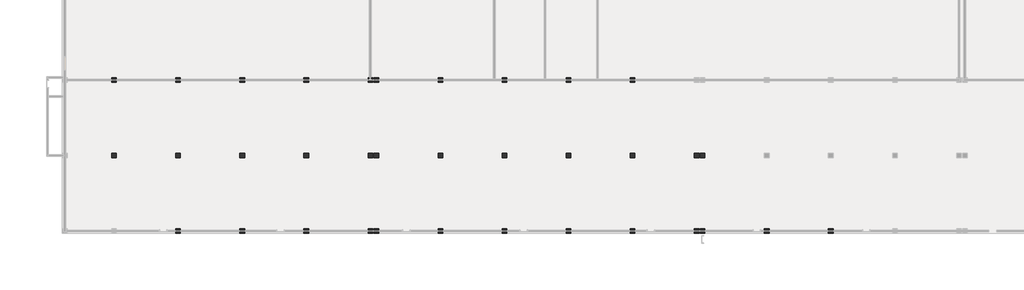
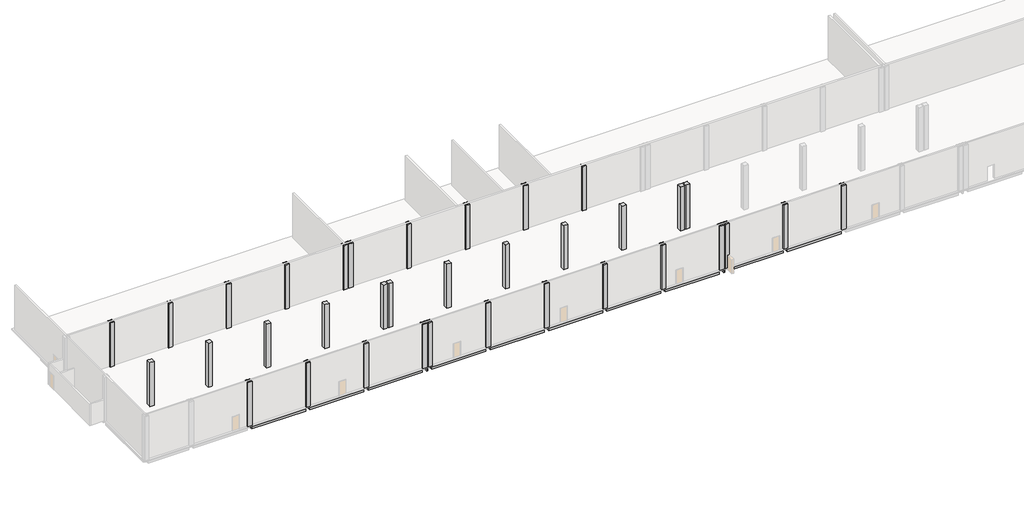
# One storey, part 2 of 4: 35 columns, 12 beams.
"""IFC4 building model written with IfcOpenShell, lengths in millimetres."""

import ifcopenshell
import ifcopenshell.guid

model = None  # the IFC model being written
_history = None  # IfcOwnerHistory: only IFC2X3 demands one
_inside = {}  # id of a spatial element -> (the spatial element, [elements in it])
_under = {}  # id of a project, library or spatial element -> (it, [spatial elements below it])
_declared = {}  # id of a project -> (the project, [libraries it declares])
_typed = {}  # id of a type object -> (the type object, [elements of that type])
_made_of = {}  # id of a material, layer set ... -> (it, [elements and type objects made of it])


def new_model(schema):
    """Start an empty IFC model of exactly this schema.

    Asked for "IFC4X3", IfcOpenShell would pick the latest addendum, in which some entities
    have other attributes; the version numbers below select the first issue.
    IFC2X3 requires an IfcOwnerHistory on every rooted entity: one is made here for all.
    """
    global model, _history
    if schema == "IFC4X3":
        model = ifcopenshell.file(schema_version=(4, 3, 0, 0))
    else:
        model = ifcopenshell.file(schema=schema)
    _inside.clear()
    _under.clear()
    _declared.clear()
    _typed.clear()
    _made_of.clear()
    _history = None
    if model.schema == "IFC2X3":
        org = make("IfcOrganization", Name="unknown")
        user = make(
            "IfcPersonAndOrganization",
            ThePerson=make("IfcPerson", FamilyName="unknown"),
            TheOrganization=org,
        )
        app = make(
            "IfcApplication",
            ApplicationDeveloper=org,
            Version="unknown",
            ApplicationFullName="unknown",
            ApplicationIdentifier="unknown",
        )
        _history = make(
            "IfcOwnerHistory",
            OwningUser=user,
            OwningApplication=app,
            ChangeAction="ADDED",
            CreationDate=0,
        )
    return model


def make(cls, **values):
    """One entity of the class cls with the attributes given. An attribute that is None is left unset."""
    return model.create_entity(
        cls, **{name: value for name, value in values.items() if value is not None}
    )


def rooted(cls, **values):
    """An entity with a GlobalId (a new one), such as an element, a storey or a relation."""
    return make(cls, GlobalId=ifcopenshell.guid.new(), OwnerHistory=_history, **values)


def si_unit(unit_type, name, prefix=None):
    """IfcSIUnit, for example si_unit("LENGTHUNIT", "METRE", prefix="MILLI")."""
    return make("IfcSIUnit", UnitType=unit_type, Prefix=prefix, Name=name)


def assignment(units):
    """IfcUnitAssignment: the units of a project."""
    return None if units is None else make("IfcUnitAssignment", Units=units)


def point(xyz):
    """IfcCartesianPoint."""
    return None if xyz is None else make("IfcCartesianPoint", Coordinates=xyz)


def direction(xyz):
    """IfcDirection."""
    return None if xyz is None else make("IfcDirection", DirectionRatios=xyz)


def frame(location, z_axis=None, x_axis=None):
    """IfcAxis2Placement3D, a coordinate frame: its origin and axes. An axis left out is left unset."""
    return make(
        "IfcAxis2Placement3D",
        Location=point(location),
        Axis=direction(z_axis),
        RefDirection=direction(x_axis),
    )


def origin():
    """The frame at (0, 0, 0) with its axes left unset."""
    return frame((0.0, 0.0, 0.0))


def place(relative_to, where):
    """IfcLocalPlacement: puts the frame where relative to a parent placement (None: the world)."""
    return make(
        "IfcLocalPlacement", PlacementRelTo=relative_to, RelativePlacement=where
    )


def context(
    kind, dimensions, precision=None, world=None, true_north=None, identifier=None
):
    """IfcGeometricRepresentationContext, for example the 3D "Model" context."""
    return make(
        "IfcGeometricRepresentationContext",
        ContextIdentifier=identifier,
        ContextType=kind,
        CoordinateSpaceDimension=dimensions,
        Precision=precision,
        WorldCoordinateSystem=world,
        TrueNorth=true_north,
    )


def project(units=None, contexts=None):
    """IfcProject with its units and contexts."""
    return rooted(
        "IfcProject",
        Name="project",
        RepresentationContexts=contexts,
        UnitsInContext=assignment(units),
    )


def spatial(cls, under=None, at=None, **own):
    """A site, building, storey or space (cls), placed at a placement, below another one or the project."""
    s = rooted(cls, ObjectPlacement=at, **own)
    if under is not None:
        _under.setdefault(under.id(), (under, []))[1].append(s)
    return s


def polyline(points):
    """IfcPolyline through the points."""
    return make("IfcPolyline", Points=[point(p) for p in points])


def outline(outer, holes=None, kind="AREA"):
    """IfcArbitraryClosedProfileDef: a profile drawn as a closed curve; with holes, ...WithVoids."""
    if holes is None:
        return make("IfcArbitraryClosedProfileDef", ProfileType=kind, OuterCurve=outer)
    return make(
        "IfcArbitraryProfileDefWithVoids",
        ProfileType=kind,
        OuterCurve=outer,
        InnerCurves=holes,
    )


def extrude(swept, where, along, depth):
    """IfcExtrudedAreaSolid: the profile swept, set in the frame where, extruded along a direction by depth."""
    return make(
        "IfcExtrudedAreaSolid",
        SweptArea=swept,
        Position=where,
        ExtrudedDirection=direction(along),
        Depth=depth,
    )


def faces_of(points, faces, orient=None, outer=None):
    """IfcFace entities. A face is a list of loops; a loop is a list of indices into points, from 0.

    orient and outer hold one flag for each loop. By default every Orientation is true, the
    first loop of a face is its IfcFaceOuterBound and the others are IfcFaceBound.
    """
    made = []
    for i, loops in enumerate(faces):
        bounds = []
        for j, loop in enumerate(loops):
            is_outer = j == 0 if outer is None else outer[i][j]
            bounds.append(
                make(
                    "IfcFaceOuterBound" if is_outer else "IfcFaceBound",
                    Bound=make("IfcPolyLoop", Polygon=[points[k] for k in loop]),
                    Orientation=True if orient is None else orient[i][j],
                )
            )
        made.append(make("IfcFace", Bounds=bounds))
    return made


def faceted_brep(points, faces, orient=None, outer=None, voids=None):
    """IfcFacetedBrep: a solid bounded by flat faces; with voids (closed shells), ...WithVoids."""
    shared = [point(p) for p in points]
    hull = make("IfcClosedShell", CfsFaces=faces_of(shared, faces, orient, outer))
    if voids is None:
        return make("IfcFacetedBrep", Outer=hull)
    return make(
        "IfcFacetedBrepWithVoids",
        Outer=hull,
        Voids=[
            make(cls, CfsFaces=faces_of(shared, fs, o, b)) for cls, fs, o, b in voids
        ],
    )


def shape(context_of_items, identifier, shape_type, items):
    """IfcShapeRepresentation: the items that make up one representation, for example the "Body"."""
    return make(
        "IfcShapeRepresentation",
        ContextOfItems=context_of_items,
        RepresentationIdentifier=identifier,
        RepresentationType=shape_type,
        Items=items,
    )


def made_of(thing, what):
    """Note that an element or type object is made of a material, layer set ...; save() writes the relation."""
    if what is not None:
        _made_of.setdefault(what.id(), (what, []))[1].append(thing)
    return thing


def element(
    cls,
    number,
    at=None,
    inside=None,
    cuts=None,
    type_object=None,
    material=None,
    context=None,
    identifier="Body",
    shape_type=None,
    held_by="IfcProductDefinitionShape",
    body=None,
    shapes=None,
    **own,
):
    """One element of the class cls, such as IfcWall. Its Tag is "e" and its number.

    at: its placement. inside: the storey or other place that contains it. cuts: it is an
    opening in that element (IfcRelVoidsElement). A single representation is given by context,
    identifier, shape_type and body (its items); several are given by shapes. held_by: the class
    of the entity that holds the representations. save() writes the other relations.
    """
    e = rooted(cls, Tag="e%d" % number, ObjectPlacement=at, **own)
    if body is not None:
        shapes = [shape(context, identifier, shape_type, body)]
    if shapes is not None:
        e.Representation = make(held_by, Representations=shapes)
    if inside is not None:
        _inside.setdefault(inside.id(), (inside, []))[1].append(e)
    if cuts is not None:
        rooted(
            "IfcRelVoidsElement", RelatingBuildingElement=cuts, RelatedOpeningElement=e
        )
    if type_object is not None:
        _typed.setdefault(type_object.id(), (type_object, []))[1].append(e)
    return made_of(e, material)


def aggregate(whole, parts):
    """IfcRelAggregates: a whole, such as a stair, and the parts it consists of."""
    return rooted("IfcRelAggregates", RelatingObject=whole, RelatedObjects=parts)


def save(model, path):
    """Write the relations noted so far, then the file.

    IfcRelAggregates (storeys below a building ...), IfcRelContainedInSpatialStructure (elements
    in a storey), IfcRelDefinesByType, IfcRelAssociatesMaterial and IfcRelDeclares: one each for
    every whole, place, type object, material and project.
    """
    for whole, parts in _under.values():
        aggregate(whole, parts)
    for where, things in _inside.values():
        rooted(
            "IfcRelContainedInSpatialStructure",
            RelatedElements=things,
            RelatingStructure=where,
        )
    for kind, things in _typed.values():
        rooted("IfcRelDefinesByType", RelatedObjects=things, RelatingType=kind)
    for what, things in _made_of.values():
        rooted("IfcRelAssociatesMaterial", RelatedObjects=things, RelatingMaterial=what)
    for by, libraries in _declared.values():
        rooted("IfcRelDeclares", RelatingContext=by, RelatedDefinitions=libraries)
    model.write(path)


model = new_model("IFC4")

# Units and contexts
model_context = context("Model", 3, world=origin())
ifc_project = project(units=[si_unit("LENGTHUNIT", "METRE", prefix="MILLI")], contexts=[model_context])

# Site, building, storey
site = spatial("IfcSite", under=ifc_project)
building = spatial("IfcBuilding", under=site)
storey = spatial("IfcBuildingStorey", under=building, Name="01_T.O.F", Elevation=299.9618634)

# Beams
placement = place(None, origin())
element("IfcBeam", 1, ObjectType="RC Beam_Rectangular : H_SB_AR_S16_TG_B400xH600", at=placement, inside=storey, context=model_context, shape_type="SweptSolid", body=[
    extrude(outline(polyline([(10430.0, -25475.4791411), (10430.0, -25125.4791411), (18030.0, -25125.4791411), (18030.0, -25475.4791411), (10430.0, -25475.4791411)])), frame((0.0, 0.0, -300.0381366), z_axis=(0.0, 0.0, 1.0), x_axis=(1.0, 0.0, 0.0)), (0.0, 0.0, 1.0), 450.0),
])
element("IfcBeam", 2, ObjectType="RC Beam_Rectangular : H_SB_AR_S16_TG_B400xH600", at=placement, inside=storey, context=model_context, shape_type="SweptSolid", body=[
    extrude(outline(polyline([(18630.0, -25475.4791411), (18630.0, -25125.4791411), (26230.0, -25125.4791411), (26230.0, -25475.4791411), (18630.0, -25475.4791411)])), frame((0.0, 0.0, -300.0381366), z_axis=(0.0, 0.0, 1.0), x_axis=(1.0, 0.0, 0.0)), (0.0, 0.0, 1.0), 450.0),
])
element("IfcBeam", 3, ObjectType="RC Beam_Rectangular : H_SB_AR_S16_TG_B400xH600", at=placement, inside=storey, context=model_context, shape_type="SweptSolid", body=[
    extrude(outline(polyline([(26830.0, -25475.4791411), (26830.0, -25125.4791411), (34430.0, -25125.4791411), (34430.0, -25475.4791411), (26830.0, -25475.4791411)])), frame((0.0, 0.0, -300.0381366), z_axis=(0.0, 0.0, 1.0), x_axis=(1.0, 0.0, 0.0)), (0.0, 0.0, 1.0), 450.0),
])
element("IfcBeam", 4, ObjectType="RC Beam_Rectangular : H_SB_AR_S16_TG_B400xH600", at=placement, inside=storey, context=model_context, shape_type="SweptSolid", body=[
    extrude(outline(polyline([(35030.0, -25475.4791411), (35030.0, -25125.4791411), (35180.0, -25125.4791411), (35180.0, -25475.4791411), (35030.0, -25475.4791411)])), frame((0.0, 0.0, -300.0381366), z_axis=(0.0, 0.0, 1.0), x_axis=(1.0, 0.0, 0.0)), (0.0, 0.0, 1.0), 450.0),
])
element("IfcBeam", 5, ObjectType="RC Beam_Rectangular : H_SB_AR_S16_TG_B400xH600", at=placement, inside=storey, context=model_context, shape_type="SweptSolid", body=[
    extrude(outline(polyline([(35780.0, -25475.4791411), (35780.0, -25125.4791411), (43380.0, -25125.4791411), (43380.0, -25475.4791411), (35780.0, -25475.4791411)])), frame((0.0, 0.0, -300.0381366), z_axis=(0.0, 0.0, 1.0), x_axis=(1.0, 0.0, 0.0)), (0.0, 0.0, 1.0), 450.0),
])
element("IfcBeam", 6, ObjectType="RC Beam_Rectangular : H_SB_AR_S16_TG_B400xH600", at=placement, inside=storey, context=model_context, shape_type="SweptSolid", body=[
    extrude(outline(polyline([(43980.0, -25475.4791411), (43980.0, -25125.4791411), (51580.0, -25125.4791411), (51580.0, -25475.4791411), (43980.0, -25475.4791411)])), frame((0.0, 0.0, -300.0381366), z_axis=(0.0, 0.0, 1.0), x_axis=(1.0, 0.0, 0.0)), (0.0, 0.0, 1.0), 450.0),
])
element("IfcBeam", 7, ObjectType="RC Beam_Rectangular : H_SB_AR_S16_TG_B400xH600", at=placement, inside=storey, context=model_context, shape_type="SweptSolid", body=[
    extrude(outline(polyline([(52180.0, -25475.4791411), (52180.0, -25125.4791411), (59780.0, -25125.4791411), (59780.0, -25475.4791411), (52180.0, -25475.4791411)])), frame((0.0, 0.0, -300.0381366), z_axis=(0.0, 0.0, 1.0), x_axis=(1.0, 0.0, 0.0)), (0.0, 0.0, 1.0), 450.0),
])
element("IfcBeam", 8, ObjectType="RC Beam_Rectangular : H_SB_AR_S16_TG_B400xH600", at=placement, inside=storey, context=model_context, shape_type="SweptSolid", body=[
    extrude(outline(polyline([(60380.0, -25475.4791411), (60380.0, -25125.4791411), (67980.0, -25125.4791411), (67980.0, -25475.4791411), (60380.0, -25475.4791411)])), frame((0.0, 0.0, -300.0381366), z_axis=(0.0, 0.0, 1.0), x_axis=(1.0, 0.0, 0.0)), (0.0, 0.0, 1.0), 450.0),
])
element("IfcBeam", 9, ObjectType="RC Beam_Rectangular : H_SB_AR_S16_TG_B400xH600", at=placement, inside=storey, context=model_context, shape_type="SweptSolid", body=[
    extrude(outline(polyline([(68580.0, -25475.4791411), (68580.0, -25125.4791411), (76180.0, -25125.4791411), (76180.0, -25475.4791411), (68580.0, -25475.4791411)])), frame((0.0, 0.0, -300.0381366), z_axis=(0.0, 0.0, 1.0), x_axis=(1.0, 0.0, 0.0)), (0.0, 0.0, 1.0), 450.0),
])
element("IfcBeam", 10, ObjectType="RC Beam_Rectangular : H_SB_AR_S16_TG_B400xH600", at=placement, inside=storey, context=model_context, shape_type="SweptSolid", body=[
    extrude(outline(polyline([(76780.0, -25475.4791411), (76780.0, -25125.4791411), (76930.0, -25125.4791411), (76930.0, -25475.4791411), (76780.0, -25475.4791411)])), frame((0.0, 0.0, -300.0381366), z_axis=(0.0, 0.0, 1.0), x_axis=(1.0, 0.0, 0.0)), (0.0, 0.0, 1.0), 450.0),
])
element("IfcBeam", 11, ObjectType="RC Beam_Rectangular : H_SB_AR_S16_TG_B400xH600", at=placement, inside=storey, context=model_context, shape_type="SweptSolid", body=[
    extrude(outline(polyline([(77530.0, -25475.4791411), (77530.0, -25125.4791411), (85130.0, -25125.4791411), (85130.0, -25475.4791411), (77530.0, -25475.4791411)])), frame((0.0, 0.0, -300.0381366), z_axis=(0.0, 0.0, 1.0), x_axis=(1.0, 0.0, 0.0)), (0.0, 0.0, 1.0), 450.0),
])
element("IfcBeam", 12, ObjectType="RC Beam_Rectangular : H_SB_AR_S16_TG_B400xH600", at=placement, inside=storey, context=model_context, shape_type="SweptSolid", body=[
    extrude(outline(polyline([(85730.0, -25475.4791411), (85730.0, -25125.4791411), (93330.0, -25125.4791411), (93330.0, -25475.4791411), (85730.0, -25475.4791411)])), frame((0.0, 0.0, -300.0381366), z_axis=(0.0, 0.0, 1.0), x_axis=(1.0, 0.0, 0.0)), (0.0, 0.0, 1.0), 450.0),
])

# Columns
element("IfcColumn", 13, ObjectType="RC_Column_Rectangular : H_SC_AR_S15_W600xL600", at=placement, inside=storey, context=model_context, shape_type="Brep", body=[
    faceted_brep([(2230.0, -5700.4791411, 299.9618634), (2230.0, -6300.4791411, 299.9618634), (1630.0, -6300.4791411, 299.9618634), (1630.0, -5700.4791411, 299.9618634), (2230.0, -5700.4791411, 6848.9618634), (2230.0, -5850.4791411, 6848.9618634), (2230.0, -6150.4791411, 6848.9618634), (2230.0, -6300.4791411, 6848.9618634), (2080.0, -6300.4791411, 6848.9618634), (1780.0, -6300.4791411, 6848.9618634), (1630.0, -6300.4791411, 6848.9618634), (1630.0, -6150.4791411, 6848.9618634), (1630.0, -5850.4791411, 6848.9618634), (1630.0, -5700.4791411, 6848.9618634), (1780.0, -5700.4791411, 6848.9618634), (2080.0, -5700.4791411, 6848.9618634)], [[[0, 1, 2, 3]], [[1, 0, 4, 5, 6, 7]], [[2, 1, 7, 8, 9, 10]], [[3, 2, 10, 11, 12, 13]], [[0, 3, 13, 14, 15, 4]], [[7, 6, 5, 4, 15, 14, 13, 12, 11, 10, 9, 8]]]),
])
element("IfcColumn", 14, ObjectType="RC_Column_Rectangular : H_SC_AR_S15_W600xL600", at=placement, inside=storey, context=model_context, shape_type="Brep", body=[
    faceted_brep([(10430.0, -5700.4791411, 299.9618634), (10430.0, -6300.4791411, 299.9618634), (9830.0, -6300.4791411, 299.9618634), (9830.0, -5700.4791411, 299.9618634), (10430.0, -5700.4791411, 6848.9618634), (10430.0, -5850.4791411, 6848.9618634), (10430.0, -6150.4791411, 6848.9618634), (10430.0, -6300.4791411, 6848.9618634), (10280.0, -6300.4791411, 6848.9618634), (9980.0, -6300.4791411, 6848.9618634), (9830.0, -6300.4791411, 6848.9618634), (9830.0, -6150.4791411, 6848.9618634), (9830.0, -5850.4791411, 6848.9618634), (9830.0, -5700.4791411, 6848.9618634), (9980.0, -5700.4791411, 6848.9618634), (10280.0, -5700.4791411, 6848.9618634)], [[[0, 1, 2, 3]], [[1, 0, 4, 5, 6, 7]], [[2, 1, 7, 8, 9, 10]], [[3, 2, 10, 11, 12, 13]], [[0, 3, 13, 14, 15, 4]], [[7, 6, 5, 4, 15, 14, 13, 12, 11, 10, 9, 8]]]),
])
element("IfcColumn", 15, ObjectType="RC_Column_Rectangular : H_SC_AR_S15_W600xL600", at=placement, inside=storey, context=model_context, shape_type="Brep", body=[
    faceted_brep([(18630.0, -5700.4791411, 299.9618634), (18630.0, -6300.4791411, 299.9618634), (18030.0, -6300.4791411, 299.9618634), (18030.0, -5700.4791411, 299.9618634), (18630.0, -5700.4791411, 6848.9618634), (18630.0, -5850.4791411, 6848.9618634), (18630.0, -6150.4791411, 6848.9618634), (18630.0, -6300.4791411, 6848.9618634), (18480.0, -6300.4791411, 6848.9618634), (18180.0, -6300.4791411, 6848.9618634), (18030.0, -6300.4791411, 6848.9618634), (18030.0, -6150.4791411, 6848.9618634), (18030.0, -5850.4791411, 6848.9618634), (18030.0, -5700.4791411, 6848.9618634), (18180.0, -5700.4791411, 6848.9618634), (18480.0, -5700.4791411, 6848.9618634)], [[[0, 1, 2, 3]], [[1, 0, 4, 5, 6, 7]], [[2, 1, 7, 8, 9, 10]], [[3, 2, 10, 11, 12, 13]], [[0, 3, 13, 14, 15, 4]], [[7, 6, 5, 4, 15, 14, 13, 12, 11, 10, 9, 8]]]),
])
element("IfcColumn", 16, ObjectType="RC_Column_Rectangular : H_SC_AR_S15_W600xL600", at=placement, inside=storey, context=model_context, shape_type="Brep", body=[
    faceted_brep([(26830.0, -5700.4791411, 299.9618634), (26830.0, -6300.4791411, 299.9618634), (26230.0, -6300.4791411, 299.9618634), (26230.0, -5700.4791411, 299.9618634), (26830.0, -5700.4791411, 6848.9618634), (26830.0, -5850.4791411, 6848.9618634), (26830.0, -6150.4791411, 6848.9618634), (26830.0, -6300.4791411, 6848.9618634), (26680.0, -6300.4791411, 6848.9618634), (26380.0, -6300.4791411, 6848.9618634), (26230.0, -6300.4791411, 6848.9618634), (26230.0, -6150.4791411, 6848.9618634), (26230.0, -5850.4791411, 6848.9618634), (26230.0, -5700.4791411, 6848.9618634), (26380.0, -5700.4791411, 6848.9618634), (26680.0, -5700.4791411, 6848.9618634)], [[[0, 1, 2, 3]], [[1, 0, 4, 5, 6, 7]], [[2, 1, 7, 8, 9, 10]], [[3, 2, 10, 11, 12, 13]], [[0, 3, 13, 14, 15, 4]], [[7, 6, 5, 4, 15, 14, 13, 12, 11, 10, 9, 8]]]),
])
element("IfcColumn", 17, ObjectType="RC_Column_Rectangular : H_SC_AR_S15_W600xL600", at=placement, inside=storey, context=model_context, shape_type="Brep", body=[
    faceted_brep([(35030.0, -5700.4791411, 299.9618634), (35030.0, -6300.4791411, 299.9618634), (34430.0, -6300.4791411, 299.9618634), (34430.0, -5700.4791411, 299.9618634), (35030.0, -5700.4791411, 6848.9618634), (35030.0, -5850.4791411, 6848.9618634), (35030.0, -6150.4791411, 6848.9618634), (35030.0, -6300.4791411, 6848.9618634), (34880.0, -6300.4791411, 6848.9618634), (34580.0, -6300.4791411, 6848.9618634), (34430.0, -6300.4791411, 6848.9618634), (34430.0, -6150.4791411, 6848.9618634), (34430.0, -5850.4791411, 6848.9618634), (34430.0, -5700.4791411, 6848.9618634), (34580.0, -5700.4791411, 6848.9618634), (34880.0, -5700.4791411, 6848.9618634)], [[[0, 1, 2, 3]], [[1, 0, 4, 5, 6, 7]], [[2, 1, 7, 8, 9, 10]], [[3, 2, 10, 11, 12, 13]], [[0, 3, 13, 14, 15, 4]], [[7, 6, 5, 4, 15, 14, 13, 12, 11, 10, 9, 8]]]),
])
element("IfcColumn", 18, ObjectType="RC_Column_Rectangular : H_SC_AR_S15_W600xL600", at=placement, inside=storey, context=model_context, shape_type="Brep", body=[
    faceted_brep([(35780.0, -5700.4791411, 299.9618634), (35780.0, -6300.4791411, 299.9618634), (35180.0, -6300.4791411, 299.9618634), (35180.0, -5700.4791411, 299.9618634), (35780.0, -5700.4791411, 6848.9618634), (35780.0, -5850.4791411, 6848.9618634), (35780.0, -6150.4791411, 6848.9618634), (35780.0, -6300.4791411, 6848.9618634), (35630.0, -6300.4791411, 6848.9618634), (35330.0, -6300.4791411, 6848.9618634), (35180.0, -6300.4791411, 6848.9618634), (35180.0, -6150.4791411, 6848.9618634), (35180.0, -5850.4791411, 6848.9618634), (35180.0, -5700.4791411, 6848.9618634), (35330.0, -5700.4791411, 6848.9618634), (35630.0, -5700.4791411, 6848.9618634)], [[[0, 1, 2, 3]], [[1, 0, 4, 5, 6, 7]], [[2, 1, 7, 8, 9, 10]], [[3, 2, 10, 11, 12, 13]], [[0, 3, 13, 14, 15, 4]], [[7, 6, 5, 4, 15, 14, 13, 12, 11, 10, 9, 8]]]),
])
element("IfcColumn", 19, ObjectType="RC_Column_Rectangular : H_SC_AR_S15_W600xL600", at=placement, inside=storey, context=model_context, shape_type="Brep", body=[
    faceted_brep([(43980.0, -5700.4791411, 299.9618634), (43980.0, -6300.4791411, 299.9618634), (43380.0, -6300.4791411, 299.9618634), (43380.0, -5700.4791411, 299.9618634), (43980.0, -5700.4791411, 6848.9618634), (43980.0, -5850.4791411, 6848.9618634), (43980.0, -6150.4791411, 6848.9618634), (43980.0, -6300.4791411, 6848.9618634), (43830.0, -6300.4791411, 6848.9618634), (43530.0, -6300.4791411, 6848.9618634), (43380.0, -6300.4791411, 6848.9618634), (43380.0, -6150.4791411, 6848.9618634), (43380.0, -5850.4791411, 6848.9618634), (43380.0, -5700.4791411, 6848.9618634), (43530.0, -5700.4791411, 6848.9618634), (43830.0, -5700.4791411, 6848.9618634)], [[[0, 1, 2, 3]], [[1, 0, 4, 5, 6, 7]], [[2, 1, 7, 8, 9, 10]], [[3, 2, 10, 11, 12, 13]], [[0, 3, 13, 14, 15, 4]], [[7, 6, 5, 4, 15, 14, 13, 12, 11, 10, 9, 8]]]),
])
element("IfcColumn", 20, ObjectType="RC_Column_Rectangular : H_SC_AR_S15_W600xL600", at=placement, inside=storey, context=model_context, shape_type="Brep", body=[
    faceted_brep([(52180.0, -5700.4791411, 299.9618634), (52180.0, -6300.4791411, 299.9618634), (51580.0, -6300.4791411, 299.9618634), (51580.0, -5700.4791411, 299.9618634), (52180.0, -5700.4791411, 6848.9618634), (52180.0, -5850.4791411, 6848.9618634), (52180.0, -6150.4791411, 6848.9618634), (52180.0, -6300.4791411, 6848.9618634), (52030.0, -6300.4791411, 6848.9618634), (51730.0, -6300.4791411, 6848.9618634), (51580.0, -6300.4791411, 6848.9618634), (51580.0, -6150.4791411, 6848.9618634), (51580.0, -5850.4791411, 6848.9618634), (51580.0, -5700.4791411, 6848.9618634), (51730.0, -5700.4791411, 6848.9618634), (52030.0, -5700.4791411, 6848.9618634)], [[[0, 1, 2, 3]], [[1, 0, 4, 5, 6, 7]], [[2, 1, 7, 8, 9, 10]], [[3, 2, 10, 11, 12, 13]], [[0, 3, 13, 14, 15, 4]], [[7, 6, 5, 4, 15, 14, 13, 12, 11, 10, 9, 8]]]),
])
element("IfcColumn", 21, ObjectType="RC_Column_Rectangular : H_SC_AR_S15_W600xL600", at=placement, inside=storey, context=model_context, shape_type="Brep", body=[
    faceted_brep([(60380.0, -5700.4791411, 299.9618634), (60380.0, -6300.4791411, 299.9618634), (59780.0, -6300.4791411, 299.9618634), (59780.0, -5700.4791411, 299.9618634), (60380.0, -5700.4791411, 6848.9618634), (60380.0, -5850.4791411, 6848.9618634), (60380.0, -6150.4791411, 6848.9618634), (60380.0, -6300.4791411, 6848.9618634), (60230.0, -6300.4791411, 6848.9618634), (59930.0, -6300.4791411, 6848.9618634), (59780.0, -6300.4791411, 6848.9618634), (59780.0, -6150.4791411, 6848.9618634), (59780.0, -5850.4791411, 6848.9618634), (59780.0, -5700.4791411, 6848.9618634), (59930.0, -5700.4791411, 6848.9618634), (60230.0, -5700.4791411, 6848.9618634)], [[[0, 1, 2, 3]], [[1, 0, 4, 5, 6, 7]], [[2, 1, 7, 8, 9, 10]], [[3, 2, 10, 11, 12, 13]], [[0, 3, 13, 14, 15, 4]], [[7, 6, 5, 4, 15, 14, 13, 12, 11, 10, 9, 8]]]),
])
element("IfcColumn", 22, ObjectType="RC_Column_Rectangular : H_SC_AR_S15_W600xL600", at=placement, inside=storey, context=model_context, shape_type="Brep", body=[
    faceted_brep([(68580.0, -5700.4791411, 299.9618634), (68580.0, -6300.4791411, 299.9618634), (67980.0, -6300.4791411, 299.9618634), (67980.0, -5700.4791411, 299.9618634), (68580.0, -5700.4791411, 6848.9618634), (68580.0, -5850.4791411, 6848.9618634), (68580.0, -6150.4791411, 6848.9618634), (68580.0, -6300.4791411, 6848.9618634), (68430.0, -6300.4791411, 6848.9618634), (68130.0, -6300.4791411, 6848.9618634), (67980.0, -6300.4791411, 6848.9618634), (67980.0, -6150.4791411, 6848.9618634), (67980.0, -5850.4791411, 6848.9618634), (67980.0, -5700.4791411, 6848.9618634), (68130.0, -5700.4791411, 6848.9618634), (68430.0, -5700.4791411, 6848.9618634)], [[[0, 1, 2, 3]], [[1, 0, 4, 5, 6, 7]], [[2, 1, 7, 8, 9, 10]], [[3, 2, 10, 11, 12, 13]], [[0, 3, 13, 14, 15, 4]], [[7, 6, 5, 4, 15, 14, 13, 12, 11, 10, 9, 8]]]),
])
element("IfcColumn", 23, ObjectType="RC_Column_Rectangular : H_SC_AR_S15_W600xL600", at=placement, inside=storey, context=model_context, shape_type="Brep", body=[
    faceted_brep([(2230.0, -15350.4791411, 299.9618634), (2230.0, -15950.4791411, 299.9618634), (1630.0, -15950.4791411, 299.9618634), (1630.0, -15350.4791411, 299.9618634), (2230.0, -15350.4791411, 6848.9618634), (2230.0, -15500.4791411, 6848.9618634), (2230.0, -15800.4791411, 6848.9618634), (2230.0, -15950.4791411, 6848.9618634), (2080.0, -15950.4791411, 6848.9618634), (1780.0, -15950.4791411, 6848.9618634), (1630.0, -15950.4791411, 6848.9618634), (1630.0, -15800.4791411, 6848.9618634), (1630.0, -15500.4791411, 6848.9618634), (1630.0, -15350.4791411, 6848.9618634), (1780.0, -15350.4791411, 6848.9618634), (2080.0, -15350.4791411, 6848.9618634)], [[[0, 1, 2, 3]], [[1, 0, 4, 5, 6, 7]], [[2, 1, 7, 8, 9, 10]], [[3, 2, 10, 11, 12, 13]], [[0, 3, 13, 14, 15, 4]], [[7, 6, 5, 4, 15, 14, 13, 12, 11, 10, 9, 8]]]),
])
element("IfcColumn", 24, ObjectType="RC_Column_Rectangular : H_SC_AR_S15_W600xL600", at=placement, inside=storey, context=model_context, shape_type="Brep", body=[
    faceted_brep([(10430.0, -15350.4791411, 299.9618634), (10430.0, -15950.4791411, 299.9618634), (9830.0, -15950.4791411, 299.9618634), (9830.0, -15350.4791411, 299.9618634), (10430.0, -15350.4791411, 6848.9618634), (10430.0, -15500.4791411, 6848.9618634), (10430.0, -15800.4791411, 6848.9618634), (10430.0, -15950.4791411, 6848.9618634), (10280.0, -15950.4791411, 6848.9618634), (9980.0, -15950.4791411, 6848.9618634), (9830.0, -15950.4791411, 6848.9618634), (9830.0, -15800.4791411, 6848.9618634), (9830.0, -15500.4791411, 6848.9618634), (9830.0, -15350.4791411, 6848.9618634), (9980.0, -15350.4791411, 6848.9618634), (10280.0, -15350.4791411, 6848.9618634)], [[[0, 1, 2, 3]], [[1, 0, 4, 5, 6, 7]], [[2, 1, 7, 8, 9, 10]], [[3, 2, 10, 11, 12, 13]], [[0, 3, 13, 14, 15, 4]], [[7, 6, 5, 4, 15, 14, 13, 12, 11, 10, 9, 8]]]),
])
element("IfcColumn", 25, ObjectType="RC_Column_Rectangular : H_SC_AR_S15_W600xL600", at=placement, inside=storey, context=model_context, shape_type="Brep", body=[
    faceted_brep([(18630.0, -15350.4791411, 299.9618634), (18630.0, -15950.4791411, 299.9618634), (18030.0, -15950.4791411, 299.9618634), (18030.0, -15350.4791411, 299.9618634), (18630.0, -15350.4791411, 6848.9618634), (18630.0, -15500.4791411, 6848.9618634), (18630.0, -15800.4791411, 6848.9618634), (18630.0, -15950.4791411, 6848.9618634), (18480.0, -15950.4791411, 6848.9618634), (18180.0, -15950.4791411, 6848.9618634), (18030.0, -15950.4791411, 6848.9618634), (18030.0, -15800.4791411, 6848.9618634), (18030.0, -15500.4791411, 6848.9618634), (18030.0, -15350.4791411, 6848.9618634), (18180.0, -15350.4791411, 6848.9618634), (18480.0, -15350.4791411, 6848.9618634)], [[[0, 1, 2, 3]], [[1, 0, 4, 5, 6, 7]], [[2, 1, 7, 8, 9, 10]], [[3, 2, 10, 11, 12, 13]], [[0, 3, 13, 14, 15, 4]], [[7, 6, 5, 4, 15, 14, 13, 12, 11, 10, 9, 8]]]),
])
element("IfcColumn", 26, ObjectType="RC_Column_Rectangular : H_SC_AR_S15_W600xL600", at=placement, inside=storey, context=model_context, shape_type="Brep", body=[
    faceted_brep([(26830.0, -15350.4791411, 299.9618634), (26830.0, -15950.4791411, 299.9618634), (26230.0, -15950.4791411, 299.9618634), (26230.0, -15350.4791411, 299.9618634), (26830.0, -15350.4791411, 6848.9618634), (26830.0, -15500.4791411, 6848.9618634), (26830.0, -15800.4791411, 6848.9618634), (26830.0, -15950.4791411, 6848.9618634), (26680.0, -15950.4791411, 6848.9618634), (26380.0, -15950.4791411, 6848.9618634), (26230.0, -15950.4791411, 6848.9618634), (26230.0, -15800.4791411, 6848.9618634), (26230.0, -15500.4791411, 6848.9618634), (26230.0, -15350.4791411, 6848.9618634), (26380.0, -15350.4791411, 6848.9618634), (26680.0, -15350.4791411, 6848.9618634)], [[[0, 1, 2, 3]], [[1, 0, 4, 5, 6, 7]], [[2, 1, 7, 8, 9, 10]], [[3, 2, 10, 11, 12, 13]], [[0, 3, 13, 14, 15, 4]], [[7, 6, 5, 4, 15, 14, 13, 12, 11, 10, 9, 8]]]),
])
element("IfcColumn", 27, ObjectType="RC_Column_Rectangular : H_SC_AR_S15_W600xL600", at=placement, inside=storey, context=model_context, shape_type="Brep", body=[
    faceted_brep([(35030.0, -15350.4791411, 299.9618634), (35030.0, -15950.4791411, 299.9618634), (34430.0, -15950.4791411, 299.9618634), (34430.0, -15350.4791411, 299.9618634), (35030.0, -15350.4791411, 6848.9618634), (35030.0, -15500.4791411, 6848.9618634), (35030.0, -15800.4791411, 6848.9618634), (35030.0, -15950.4791411, 6848.9618634), (34880.0, -15950.4791411, 6848.9618634), (34580.0, -15950.4791411, 6848.9618634), (34430.0, -15950.4791411, 6848.9618634), (34430.0, -15800.4791411, 6848.9618634), (34430.0, -15500.4791411, 6848.9618634), (34430.0, -15350.4791411, 6848.9618634), (34580.0, -15350.4791411, 6848.9618634), (34880.0, -15350.4791411, 6848.9618634)], [[[0, 1, 2, 3]], [[1, 0, 4, 5, 6, 7]], [[2, 1, 7, 8, 9, 10]], [[3, 2, 10, 11, 12, 13]], [[0, 3, 13, 14, 15, 4]], [[7, 6, 5, 4, 15, 14, 13, 12, 11, 10, 9, 8]]]),
])
element("IfcColumn", 28, ObjectType="RC_Column_Rectangular : H_SC_AR_S15_W600xL600", at=placement, inside=storey, context=model_context, shape_type="Brep", body=[
    faceted_brep([(35780.0, -15350.4791411, 299.9618634), (35780.0, -15950.4791411, 299.9618634), (35180.0, -15950.4791411, 299.9618634), (35180.0, -15350.4791411, 299.9618634), (35780.0, -15350.4791411, 6848.9618634), (35780.0, -15500.4791411, 6848.9618634), (35780.0, -15800.4791411, 6848.9618634), (35780.0, -15950.4791411, 6848.9618634), (35630.0, -15950.4791411, 6848.9618634), (35330.0, -15950.4791411, 6848.9618634), (35180.0, -15950.4791411, 6848.9618634), (35180.0, -15800.4791411, 6848.9618634), (35180.0, -15500.4791411, 6848.9618634), (35180.0, -15350.4791411, 6848.9618634), (35330.0, -15350.4791411, 6848.9618634), (35630.0, -15350.4791411, 6848.9618634)], [[[0, 1, 2, 3]], [[1, 0, 4, 5, 6, 7]], [[2, 1, 7, 8, 9, 10]], [[3, 2, 10, 11, 12, 13]], [[0, 3, 13, 14, 15, 4]], [[7, 6, 5, 4, 15, 14, 13, 12, 11, 10, 9, 8]]]),
])
element("IfcColumn", 29, ObjectType="RC_Column_Rectangular : H_SC_AR_S15_W600xL600", at=placement, inside=storey, context=model_context, shape_type="Brep", body=[
    faceted_brep([(43980.0, -15350.4791411, 299.9618634), (43980.0, -15950.4791411, 299.9618634), (43380.0, -15950.4791411, 299.9618634), (43380.0, -15350.4791411, 299.9618634), (43980.0, -15350.4791411, 6848.9618634), (43980.0, -15500.4791411, 6848.9618634), (43980.0, -15800.4791411, 6848.9618634), (43980.0, -15950.4791411, 6848.9618634), (43830.0, -15950.4791411, 6848.9618634), (43530.0, -15950.4791411, 6848.9618634), (43380.0, -15950.4791411, 6848.9618634), (43380.0, -15800.4791411, 6848.9618634), (43380.0, -15500.4791411, 6848.9618634), (43380.0, -15350.4791411, 6848.9618634), (43530.0, -15350.4791411, 6848.9618634), (43830.0, -15350.4791411, 6848.9618634)], [[[0, 1, 2, 3]], [[1, 0, 4, 5, 6, 7]], [[2, 1, 7, 8, 9, 10]], [[3, 2, 10, 11, 12, 13]], [[0, 3, 13, 14, 15, 4]], [[7, 6, 5, 4, 15, 14, 13, 12, 11, 10, 9, 8]]]),
])
element("IfcColumn", 30, ObjectType="RC_Column_Rectangular : H_SC_AR_S15_W600xL600", at=placement, inside=storey, context=model_context, shape_type="Brep", body=[
    faceted_brep([(52180.0, -15350.4791411, 299.9618634), (52180.0, -15950.4791411, 299.9618634), (51580.0, -15950.4791411, 299.9618634), (51580.0, -15350.4791411, 299.9618634), (52180.0, -15350.4791411, 6848.9618634), (52180.0, -15500.4791411, 6848.9618634), (52180.0, -15800.4791411, 6848.9618634), (52180.0, -15950.4791411, 6848.9618634), (52030.0, -15950.4791411, 6848.9618634), (51730.0, -15950.4791411, 6848.9618634), (51580.0, -15950.4791411, 6848.9618634), (51580.0, -15800.4791411, 6848.9618634), (51580.0, -15500.4791411, 6848.9618634), (51580.0, -15350.4791411, 6848.9618634), (51730.0, -15350.4791411, 6848.9618634), (52030.0, -15350.4791411, 6848.9618634)], [[[0, 1, 2, 3]], [[1, 0, 4, 5, 6, 7]], [[2, 1, 7, 8, 9, 10]], [[3, 2, 10, 11, 12, 13]], [[0, 3, 13, 14, 15, 4]], [[7, 6, 5, 4, 15, 14, 13, 12, 11, 10, 9, 8]]]),
])
element("IfcColumn", 31, ObjectType="RC_Column_Rectangular : H_SC_AR_S15_W600xL600", at=placement, inside=storey, context=model_context, shape_type="Brep", body=[
    faceted_brep([(60380.0, -15350.4791411, 299.9618634), (60380.0, -15950.4791411, 299.9618634), (59780.0, -15950.4791411, 299.9618634), (59780.0, -15350.4791411, 299.9618634), (60380.0, -15350.4791411, 6848.9618634), (60380.0, -15500.4791411, 6848.9618634), (60380.0, -15800.4791411, 6848.9618634), (60380.0, -15950.4791411, 6848.9618634), (60230.0, -15950.4791411, 6848.9618634), (59930.0, -15950.4791411, 6848.9618634), (59780.0, -15950.4791411, 6848.9618634), (59780.0, -15800.4791411, 6848.9618634), (59780.0, -15500.4791411, 6848.9618634), (59780.0, -15350.4791411, 6848.9618634), (59930.0, -15350.4791411, 6848.9618634), (60230.0, -15350.4791411, 6848.9618634)], [[[0, 1, 2, 3]], [[1, 0, 4, 5, 6, 7]], [[2, 1, 7, 8, 9, 10]], [[3, 2, 10, 11, 12, 13]], [[0, 3, 13, 14, 15, 4]], [[7, 6, 5, 4, 15, 14, 13, 12, 11, 10, 9, 8]]]),
])
element("IfcColumn", 32, ObjectType="RC_Column_Rectangular : H_SC_AR_S15_W600xL600", at=placement, inside=storey, context=model_context, shape_type="Brep", body=[
    faceted_brep([(68580.0, -15350.4791411, 299.9618634), (68580.0, -15950.4791411, 299.9618634), (67980.0, -15950.4791411, 299.9618634), (67980.0, -15350.4791411, 299.9618634), (68580.0, -15350.4791411, 6848.9618634), (68580.0, -15500.4791411, 6848.9618634), (68580.0, -15800.4791411, 6848.9618634), (68580.0, -15950.4791411, 6848.9618634), (68430.0, -15950.4791411, 6848.9618634), (68130.0, -15950.4791411, 6848.9618634), (67980.0, -15950.4791411, 6848.9618634), (67980.0, -15800.4791411, 6848.9618634), (67980.0, -15500.4791411, 6848.9618634), (67980.0, -15350.4791411, 6848.9618634), (68130.0, -15350.4791411, 6848.9618634), (68430.0, -15350.4791411, 6848.9618634)], [[[0, 1, 2, 3]], [[1, 0, 4, 5, 6, 7]], [[2, 1, 7, 8, 9, 10]], [[3, 2, 10, 11, 12, 13]], [[0, 3, 13, 14, 15, 4]], [[7, 6, 5, 4, 15, 14, 13, 12, 11, 10, 9, 8]]]),
])
element("IfcColumn", 33, ObjectType="RC_Column_Rectangular : H_SC_AR_S15_W600xL600", at=placement, inside=storey, context=model_context, shape_type="Brep", body=[
    faceted_brep([(76780.0, -15350.4791411, 299.9618634), (76780.0, -15950.4791411, 299.9618634), (76180.0, -15950.4791411, 299.9618634), (76180.0, -15350.4791411, 299.9618634), (76780.0, -15350.4791411, 6848.9618634), (76780.0, -15500.4791411, 6848.9618634), (76780.0, -15800.4791411, 6848.9618634), (76780.0, -15950.4791411, 6848.9618634), (76630.0, -15950.4791411, 6848.9618634), (76330.0, -15950.4791411, 6848.9618634), (76180.0, -15950.4791411, 6848.9618634), (76180.0, -15800.4791411, 6848.9618634), (76180.0, -15500.4791411, 6848.9618634), (76180.0, -15350.4791411, 6848.9618634), (76330.0, -15350.4791411, 6848.9618634), (76630.0, -15350.4791411, 6848.9618634)], [[[0, 1, 2, 3]], [[1, 0, 4, 5, 6, 7]], [[2, 1, 7, 8, 9, 10]], [[3, 2, 10, 11, 12, 13]], [[0, 3, 13, 14, 15, 4]], [[7, 6, 5, 4, 15, 14, 13, 12, 11, 10, 9, 8]]]),
])
element("IfcColumn", 34, ObjectType="RC_Column_Rectangular : H_SC_AR_S15_W600xL600", at=placement, inside=storey, context=model_context, shape_type="Brep", body=[
    faceted_brep([(77530.0, -15350.4791411, 299.9618634), (77530.0, -15950.4791411, 299.9618634), (76930.0, -15950.4791411, 299.9618634), (76930.0, -15350.4791411, 299.9618634), (77530.0, -15350.4791411, 6848.9618634), (77530.0, -15500.4791411, 6848.9618634), (77530.0, -15800.4791411, 6848.9618634), (77530.0, -15950.4791411, 6848.9618634), (77380.0, -15950.4791411, 6848.9618634), (77080.0, -15950.4791411, 6848.9618634), (76930.0, -15950.4791411, 6848.9618634), (76930.0, -15800.4791411, 6848.9618634), (76930.0, -15500.4791411, 6848.9618634), (76930.0, -15350.4791411, 6848.9618634), (77080.0, -15350.4791411, 6848.9618634), (77380.0, -15350.4791411, 6848.9618634)], [[[0, 1, 2, 3]], [[1, 0, 4, 5, 6, 7]], [[2, 1, 7, 8, 9, 10]], [[3, 2, 10, 11, 12, 13]], [[0, 3, 13, 14, 15, 4]], [[7, 6, 5, 4, 15, 14, 13, 12, 11, 10, 9, 8]]]),
])
element("IfcColumn", 35, ObjectType="RC_Column_Rectangular : H_SC_AR_S15_W600xL600", at=placement, inside=storey, context=model_context, shape_type="Brep", body=[
    faceted_brep([(10430.0, -25000.4791411, 299.9618634), (10430.0, -25600.4791411, 299.9618634), (9830.0, -25600.4791411, 299.9618634), (9830.0, -25000.4791411, 299.9618634), (10430.0, -25000.4791411, 6848.9618634), (10430.0, -25150.4791411, 6848.9618634), (10430.0, -25450.4791411, 6848.9618634), (10430.0, -25600.4791411, 6848.9618634), (9830.0, -25600.4791411, 6848.9618634), (9830.0, -25450.4791411, 6848.9618634), (9830.0, -25150.4791411, 6848.9618634), (9830.0, -25000.4791411, 6848.9618634), (9980.0, -25000.4791411, 6848.9618634), (10280.0, -25000.4791411, 6848.9618634)], [[[0, 1, 2, 3]], [[1, 0, 4, 5, 6, 7]], [[2, 1, 7, 8]], [[3, 2, 8, 9, 10, 11]], [[0, 3, 11, 12, 13, 4]], [[7, 6, 5, 4, 13, 12, 11, 10, 9, 8]]]),
])
element("IfcColumn", 36, ObjectType="RC_Column_Rectangular : H_SC_AR_S15_W600xL600", at=placement, inside=storey, context=model_context, shape_type="Brep", body=[
    faceted_brep([(18630.0, -25000.4791411, 299.9618634), (18630.0, -25600.4791411, 299.9618634), (18030.0, -25600.4791411, 299.9618634), (18030.0, -25000.4791411, 299.9618634), (18630.0, -25000.4791411, 6848.9618634), (18630.0, -25150.4791411, 6848.9618634), (18630.0, -25450.4791411, 6848.9618634), (18630.0, -25600.4791411, 6848.9618634), (18030.0, -25600.4791411, 6848.9618634), (18030.0, -25450.4791411, 6848.9618634), (18030.0, -25150.4791411, 6848.9618634), (18030.0, -25000.4791411, 6848.9618634), (18180.0, -25000.4791411, 6848.9618634), (18480.0, -25000.4791411, 6848.9618634)], [[[0, 1, 2, 3]], [[1, 0, 4, 5, 6, 7]], [[2, 1, 7, 8]], [[3, 2, 8, 9, 10, 11]], [[0, 3, 11, 12, 13, 4]], [[7, 6, 5, 4, 13, 12, 11, 10, 9, 8]]]),
])
element("IfcColumn", 37, ObjectType="RC_Column_Rectangular : H_SC_AR_S15_W600xL600", at=placement, inside=storey, context=model_context, shape_type="Brep", body=[
    faceted_brep([(26830.0, -25000.4791411, 299.9618634), (26830.0, -25600.4791411, 299.9618634), (26230.0, -25600.4791411, 299.9618634), (26230.0, -25000.4791411, 299.9618634), (26830.0, -25000.4791411, 6848.9618634), (26830.0, -25150.4791411, 6848.9618634), (26830.0, -25450.4791411, 6848.9618634), (26830.0, -25600.4791411, 6848.9618634), (26230.0, -25600.4791411, 6848.9618634), (26230.0, -25450.4791411, 6848.9618634), (26230.0, -25150.4791411, 6848.9618634), (26230.0, -25000.4791411, 6848.9618634), (26380.0, -25000.4791411, 6848.9618634), (26680.0, -25000.4791411, 6848.9618634)], [[[0, 1, 2, 3]], [[1, 0, 4, 5, 6, 7]], [[2, 1, 7, 8]], [[3, 2, 8, 9, 10, 11]], [[0, 3, 11, 12, 13, 4]], [[7, 6, 5, 4, 13, 12, 11, 10, 9, 8]]]),
])
element("IfcColumn", 38, ObjectType="RC_Column_Rectangular : H_SC_AR_S15_W600xL600", at=placement, inside=storey, context=model_context, shape_type="Brep", body=[
    faceted_brep([(35030.0, -25000.4791411, 299.9618634), (35030.0, -25600.4791411, 299.9618634), (34430.0, -25600.4791411, 299.9618634), (34430.0, -25000.4791411, 299.9618634), (35030.0, -25000.4791411, 6848.9618634), (35030.0, -25150.4791411, 6848.9618634), (35030.0, -25450.4791411, 6848.9618634), (35030.0, -25600.4791411, 6848.9618634), (34430.0, -25600.4791411, 6848.9618634), (34430.0, -25450.4791411, 6848.9618634), (34430.0, -25150.4791411, 6848.9618634), (34430.0, -25000.4791411, 6848.9618634), (34580.0, -25000.4791411, 6848.9618634), (34880.0, -25000.4791411, 6848.9618634)], [[[0, 1, 2, 3]], [[1, 0, 4, 5, 6, 7]], [[2, 1, 7, 8]], [[3, 2, 8, 9, 10, 11]], [[0, 3, 11, 12, 13, 4]], [[7, 6, 5, 4, 13, 12, 11, 10, 9, 8]]]),
])
element("IfcColumn", 39, ObjectType="RC_Column_Rectangular : H_SC_AR_S15_W600xL600", at=placement, inside=storey, context=model_context, shape_type="Brep", body=[
    faceted_brep([(35780.0, -25000.4791411, 299.9618634), (35780.0, -25600.4791411, 299.9618634), (35180.0, -25600.4791411, 299.9618634), (35180.0, -25000.4791411, 299.9618634), (35780.0, -25000.4791411, 6848.9618634), (35780.0, -25150.4791411, 6848.9618634), (35780.0, -25450.4791411, 6848.9618634), (35780.0, -25600.4791411, 6848.9618634), (35180.0, -25600.4791411, 6848.9618634), (35180.0, -25450.4791411, 6848.9618634), (35180.0, -25150.4791411, 6848.9618634), (35180.0, -25000.4791411, 6848.9618634), (35330.0, -25000.4791411, 6848.9618634), (35630.0, -25000.4791411, 6848.9618634)], [[[0, 1, 2, 3]], [[1, 0, 4, 5, 6, 7]], [[2, 1, 7, 8]], [[3, 2, 8, 9, 10, 11]], [[0, 3, 11, 12, 13, 4]], [[7, 6, 5, 4, 13, 12, 11, 10, 9, 8]]]),
])
element("IfcColumn", 40, ObjectType="RC_Column_Rectangular : H_SC_AR_S15_W600xL600", at=placement, inside=storey, context=model_context, shape_type="Brep", body=[
    faceted_brep([(43980.0, -25000.4791411, 299.9618634), (43980.0, -25600.4791411, 299.9618634), (43380.0, -25600.4791411, 299.9618634), (43380.0, -25000.4791411, 299.9618634), (43980.0, -25000.4791411, 6848.9618634), (43980.0, -25150.4791411, 6848.9618634), (43980.0, -25450.4791411, 6848.9618634), (43980.0, -25600.4791411, 6848.9618634), (43380.0, -25600.4791411, 6848.9618634), (43380.0, -25450.4791411, 6848.9618634), (43380.0, -25150.4791411, 6848.9618634), (43380.0, -25000.4791411, 6848.9618634), (43530.0, -25000.4791411, 6848.9618634), (43830.0, -25000.4791411, 6848.9618634)], [[[0, 1, 2, 3]], [[1, 0, 4, 5, 6, 7]], [[2, 1, 7, 8]], [[3, 2, 8, 9, 10, 11]], [[0, 3, 11, 12, 13, 4]], [[7, 6, 5, 4, 13, 12, 11, 10, 9, 8]]]),
])
element("IfcColumn", 41, ObjectType="RC_Column_Rectangular : H_SC_AR_S15_W600xL600", at=placement, inside=storey, context=model_context, shape_type="Brep", body=[
    faceted_brep([(52180.0, -25000.4791411, 299.9618634), (52180.0, -25600.4791411, 299.9618634), (51580.0, -25600.4791411, 299.9618634), (51580.0, -25000.4791411, 299.9618634), (52180.0, -25000.4791411, 6848.9618634), (52180.0, -25150.4791411, 6848.9618634), (52180.0, -25450.4791411, 6848.9618634), (52180.0, -25600.4791411, 6848.9618634), (51580.0, -25600.4791411, 6848.9618634), (51580.0, -25450.4791411, 6848.9618634), (51580.0, -25150.4791411, 6848.9618634), (51580.0, -25000.4791411, 6848.9618634), (51730.0, -25000.4791411, 6848.9618634), (52030.0, -25000.4791411, 6848.9618634)], [[[0, 1, 2, 3]], [[1, 0, 4, 5, 6, 7]], [[2, 1, 7, 8]], [[3, 2, 8, 9, 10, 11]], [[0, 3, 11, 12, 13, 4]], [[7, 6, 5, 4, 13, 12, 11, 10, 9, 8]]]),
])
element("IfcColumn", 42, ObjectType="RC_Column_Rectangular : H_SC_AR_S15_W600xL600", at=placement, inside=storey, context=model_context, shape_type="Brep", body=[
    faceted_brep([(60380.0, -25000.4791411, 299.9618634), (60380.0, -25600.4791411, 299.9618634), (59780.0, -25600.4791411, 299.9618634), (59780.0, -25000.4791411, 299.9618634), (60380.0, -25000.4791411, 6848.9618634), (60380.0, -25150.4791411, 6848.9618634), (60380.0, -25450.4791411, 6848.9618634), (60380.0, -25600.4791411, 6848.9618634), (59780.0, -25600.4791411, 6848.9618634), (59780.0, -25450.4791411, 6848.9618634), (59780.0, -25150.4791411, 6848.9618634), (59780.0, -25000.4791411, 6848.9618634), (59930.0, -25000.4791411, 6848.9618634), (60230.0, -25000.4791411, 6848.9618634)], [[[0, 1, 2, 3]], [[1, 0, 4, 5, 6, 7]], [[2, 1, 7, 8]], [[3, 2, 8, 9, 10, 11]], [[0, 3, 11, 12, 13, 4]], [[7, 6, 5, 4, 13, 12, 11, 10, 9, 8]]]),
])
element("IfcColumn", 43, ObjectType="RC_Column_Rectangular : H_SC_AR_S15_W600xL600", at=placement, inside=storey, context=model_context, shape_type="Brep", body=[
    faceted_brep([(68580.0, -25000.4791411, 299.9618634), (68580.0, -25600.4791411, 299.9618634), (67980.0, -25600.4791411, 299.9618634), (67980.0, -25000.4791411, 299.9618634), (68580.0, -25000.4791411, 6848.9618634), (68580.0, -25150.4791411, 6848.9618634), (68580.0, -25450.4791411, 6848.9618634), (68580.0, -25600.4791411, 6848.9618634), (67980.0, -25600.4791411, 6848.9618634), (67980.0, -25450.4791411, 6848.9618634), (67980.0, -25150.4791411, 6848.9618634), (67980.0, -25000.4791411, 6848.9618634), (68130.0, -25000.4791411, 6848.9618634), (68430.0, -25000.4791411, 6848.9618634)], [[[0, 1, 2, 3]], [[1, 0, 4, 5, 6, 7]], [[2, 1, 7, 8]], [[3, 2, 8, 9, 10, 11]], [[0, 3, 11, 12, 13, 4]], [[7, 6, 5, 4, 13, 12, 11, 10, 9, 8]]]),
])
element("IfcColumn", 44, ObjectType="RC_Column_Rectangular : H_SC_AR_S15_W600xL600", at=placement, inside=storey, context=model_context, shape_type="Brep", body=[
    faceted_brep([(76780.0, -25000.4791411, 299.9618634), (76780.0, -25600.4791411, 299.9618634), (76180.0, -25600.4791411, 299.9618634), (76180.0, -25000.4791411, 299.9618634), (76780.0, -25000.4791411, 6848.9618634), (76780.0, -25150.4791411, 6848.9618634), (76780.0, -25450.4791411, 6848.9618634), (76780.0, -25600.4791411, 6848.9618634), (76180.0, -25600.4791411, 6848.9618634), (76180.0, -25450.4791411, 6848.9618634), (76180.0, -25150.4791411, 6848.9618634), (76180.0, -25000.4791411, 6848.9618634), (76330.0, -25000.4791411, 6848.9618634), (76630.0, -25000.4791411, 6848.9618634)], [[[0, 1, 2, 3]], [[1, 0, 4, 5, 6, 7]], [[2, 1, 7, 8]], [[3, 2, 8, 9, 10, 11]], [[0, 3, 11, 12, 13, 4]], [[7, 6, 5, 4, 13, 12, 11, 10, 9, 8]]]),
])
element("IfcColumn", 45, ObjectType="RC_Column_Rectangular : H_SC_AR_S15_W600xL600", at=placement, inside=storey, context=model_context, shape_type="Brep", body=[
    faceted_brep([(77530.0, -25000.4791411, 299.9618634), (77530.0, -25600.4791411, 299.9618634), (76930.0, -25600.4791411, 299.9618634), (76930.0, -25000.4791411, 299.9618634), (77530.0, -25000.4791411, 6848.9618634), (77530.0, -25150.4791411, 6848.9618634), (77530.0, -25450.4791411, 6848.9618634), (77530.0, -25600.4791411, 6848.9618634), (76930.0, -25600.4791411, 6848.9618634), (76930.0, -25450.4791411, 6848.9618634), (76930.0, -25150.4791411, 6848.9618634), (76930.0, -25000.4791411, 6848.9618634), (77080.0, -25000.4791411, 6848.9618634), (77380.0, -25000.4791411, 6848.9618634)], [[[0, 1, 2, 3]], [[1, 0, 4, 5, 6, 7]], [[2, 1, 7, 8]], [[3, 2, 8, 9, 10, 11]], [[0, 3, 11, 12, 13, 4]], [[7, 6, 5, 4, 13, 12, 11, 10, 9, 8]]]),
])
element("IfcColumn", 46, ObjectType="RC_Column_Rectangular : H_SC_AR_S15_W600xL600", at=placement, inside=storey, context=model_context, shape_type="Brep", body=[
    faceted_brep([(85730.0, -25000.4791411, 299.9618634), (85730.0, -25600.4791411, 299.9618634), (85130.0, -25600.4791411, 299.9618634), (85130.0, -25000.4791411, 299.9618634), (85730.0, -25000.4791411, 6848.9618634), (85730.0, -25150.4791411, 6848.9618634), (85730.0, -25450.4791411, 6848.9618634), (85730.0, -25600.4791411, 6848.9618634), (85130.0, -25600.4791411, 6848.9618634), (85130.0, -25450.4791411, 6848.9618634), (85130.0, -25150.4791411, 6848.9618634), (85130.0, -25000.4791411, 6848.9618634), (85280.0, -25000.4791411, 6848.9618634), (85580.0, -25000.4791411, 6848.9618634)], [[[0, 1, 2, 3]], [[1, 0, 4, 5, 6, 7]], [[2, 1, 7, 8]], [[3, 2, 8, 9, 10, 11]], [[0, 3, 11, 12, 13, 4]], [[7, 6, 5, 4, 13, 12, 11, 10, 9, 8]]]),
])
element("IfcColumn", 47, ObjectType="RC_Column_Rectangular : H_SC_AR_S15_W600xL600", at=placement, inside=storey, context=model_context, shape_type="Brep", body=[
    faceted_brep([(93930.0, -25000.4791411, 299.9618634), (93930.0, -25600.4791411, 299.9618634), (93330.0, -25600.4791411, 299.9618634), (93330.0, -25000.4791411, 299.9618634), (93930.0, -25000.4791411, 6848.9618634), (93930.0, -25150.4791411, 6848.9618634), (93930.0, -25450.4791411, 6848.9618634), (93930.0, -25600.4791411, 6848.9618634), (93330.0, -25600.4791411, 6848.9618634), (93330.0, -25450.4791411, 6848.9618634), (93330.0, -25150.4791411, 6848.9618634), (93330.0, -25000.4791411, 6848.9618634), (93480.0, -25000.4791411, 6848.9618634), (93780.0, -25000.4791411, 6848.9618634)], [[[0, 1, 2, 3]], [[1, 0, 4, 5, 6, 7]], [[2, 1, 7, 8]], [[3, 2, 8, 9, 10, 11]], [[0, 3, 11, 12, 13, 4]], [[7, 6, 5, 4, 13, 12, 11, 10, 9, 8]]]),
])

save(model, "model.ifc")

# Revit data of these elements
# Type "RC Beam_Rectangular : H_SB_AR_S16_TG_B400xH600"
#   중앙부 하부근 = ""
#   중앙부 상부근 = ""
#   중앙부 보조근 = ""
#   중앙부 늑근 = ""
#   외단부 하부근 = ""
#   외단부 상부근 = ""
#   외단부 보조근 = ""
#   외단부 늑근 = ""
#   부호 = "TG2"
#   내단부 하부근 = ""
#   내단부 상부근 = ""
#   내단부 보조근 = ""
#   내단부 늑근 = ""
#   ALL 하부근 = "3-D20"
#   ALL 상부근 = "4-D20"
#   ALL 보조근 = ""
#   ALL 늑근 = "2-D10 @120"
#   Width = 350 mm
#   Height = 600 mm
#   Length [instance default] = 1524 mm
#   b = 350 mm
#   h = 600 mm
#   hec_material3 [instance default] = none
#   hec_material2 [instance default] = none
#   hec_material1 [instance default] = none
#   Structural Material [instance default] = none
#   Assembly Code = ""
# Type "RC_Column_Rectangular : H_SC_AR_S15_W600xL600"
#   Width = 600 mm
#   Length = 600 mm
#   hec_material3 [instance default] = none
#   hec_material2 [instance default] = none
#   hec_material1 [instance default] = none
#   Structural Material [instance default] = none
#   Description = (empty or 0)
# Elements 1, 2, 3, 4, 5, 6, 7, 8, 9, 10, 11, 12 (IfcBeam, "RC Beam_Rectangular : H_SB_AR_S16_TG_B400xH600")
#   Comments = ""
#   hec_material3 = none
#   hec_material2 = none
#   hec_material1 = none
#   Structural Material = none
#   Phase Created = New Construction
# Elements 13, 14, 15, 16, 17, 18, 19, 20, 21, 22, 23, 24, 25, 26, 27, 28, 29, 30, 31, 32, 33, 34, 35, 36, 37, 38, 39, 40, 41, 42, 43, 44, 45, 46, 47 (IfcColumn, "RC_Column_Rectangular : H_SC_AR_S15_W600xL600")
#   Comments = ""
#   hec_material3 = none
#   hec_material2 = none
#   hec_material1 = none
#   Structural Material = none
#   Phase Created = New Construction
